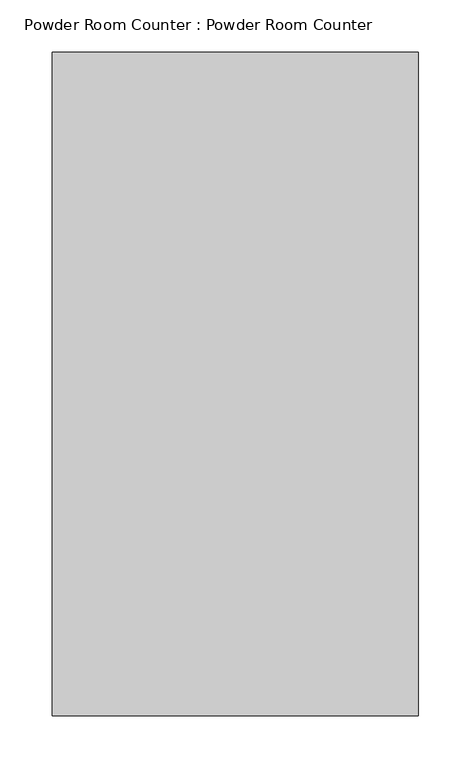
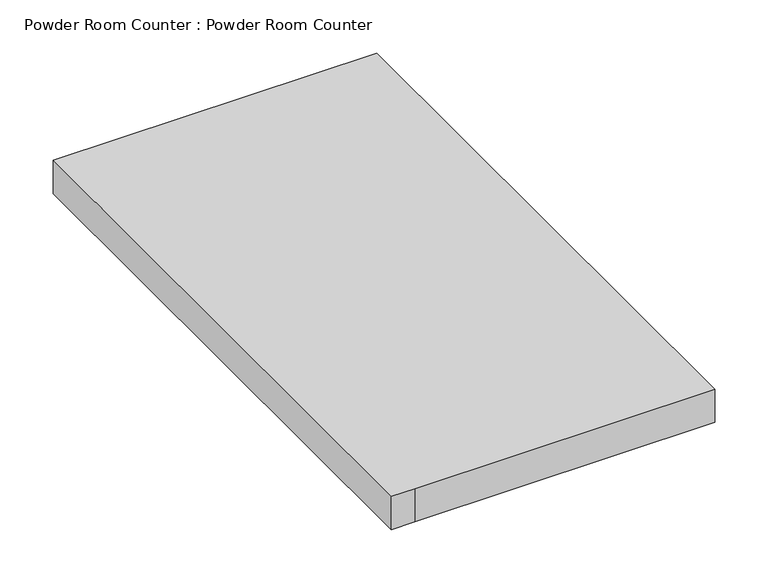
"""IFC4 building model written with IfcOpenShell, lengths in millimetres: furniture geometry, Powder Room Counter : Powder Room Counter."""

from ifc_helpers import new_model, si_unit, frame, origin, place, context, project, spatial, polyline, outline, extrude, source, transform, mapped, element, save


def powder_room_counter_powder_room_counter_269541ac(model_context):
    return source(origin(), model_context, "Body", "SweptSolid", [
        extrude(outline(polyline([(-5379.72, 11658.6), (-5379.72, 12293.6), (-5029.2, 12293.6), (-5029.2, 11658.6), (-5354.32, 11658.6), (-5379.72, 11658.6)])), frame((0.0, 0.0, 876.3), z_axis=(0.0, 0.0, 1.0), x_axis=(1.0, 0.0, 0.0)), (0.0, 0.0, 1.0), 38.1),
    ])


if __name__ == "__main__":
    model = new_model("IFC4")
    model_context = context("Model", 3, world=origin())
    ifc_project = project(units=[si_unit("LENGTHUNIT", "METRE", prefix="MILLI")], contexts=[model_context])
    site = spatial("IfcSite", under=ifc_project)
    building = spatial("IfcBuilding", under=site)
    placement = place(None, origin())
    powder_room_counter_powder_room_counter_shape = powder_room_counter_powder_room_counter_269541ac(model_context)
    element("IfcFurniture", 1, ObjectType="Powder Room Counter : Powder Room Counter", at=placement, inside=building, context=model_context, shape_type="MappedRepresentation", body=[
        mapped(powder_room_counter_powder_room_counter_shape, transform((0.0, 0.0, 0.0), x_axis=(1.0, 0.0, 0.0), y_axis=(0.0, 1.0, 0.0), z_axis=(0.0, 0.0, 1.0))),
    ])
    save(model, "model.ifc")

# Revit data of these elements
# Type "Powder Room Counter : Powder Room Counter"
#   COBie.Type = no
# Element 1 (IfcFurniture, "Powder Room Counter : Powder Room Counter")
#   Materials on its faces: "Corian - Emerald"
# Materials
#   "Corian - Emerald": class "Plastic", colour RGB 51 95 44, transparency 0, Cost = 0
